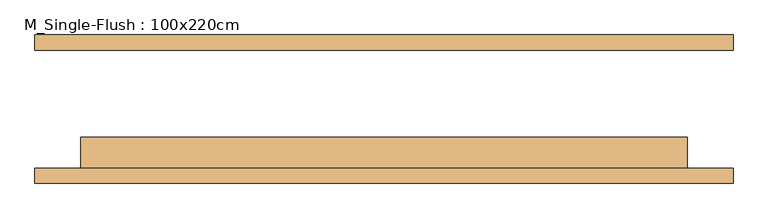
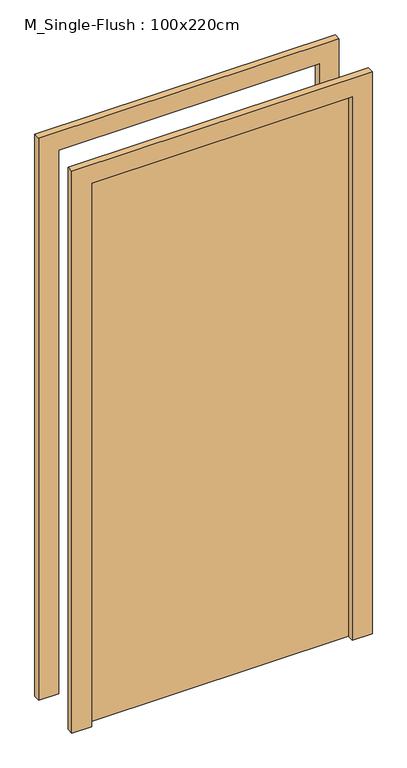
"""IFC4 building model written with IfcOpenShell, lengths in millimetres: door geometry, M_Single-Flush : 100x220cm."""

from ifc_helpers import new_model, si_unit, frame, origin, origin_with_axes, place, context, project, spatial, polyline, outline, extrude, source, transform, mapped, element, save


def m_single_flush_100x220cm_94bd71e5(model_context):
    return source(origin(), model_context, "Body", "SweptSolid", [
        extrude(outline(polyline([(2276.0, -576.0), (0.0, -576.0), (0.0, -500.0), (2200.0, -500.0), (2200.0, 500.0), (0.0, 500.0), (0.0, 576.0), (2276.0, 576.0), (2276.0, -576.0)])), frame((0.0, -122.5, 0.0), z_axis=(0.0, 1.0, 0.0), x_axis=(0.0, 0.0, 1.0)), (0.0, 0.0, 1.0), 25.0),
        extrude(outline(polyline([(2276.0, 576.0), (2276.0, -576.0), (0.0, -576.0), (0.0, -500.0), (2200.0, -500.0), (2200.0, 500.0), (0.0, 500.0), (0.0, 576.0), (2276.0, 576.0)])), frame((0.0, 97.5, 0.0), z_axis=(0.0, 1.0, 0.0), x_axis=(0.0, 0.0, 1.0)), (0.0, 0.0, 1.0), 25.0),
        extrude(outline(polyline([(500.0, -46.5), (500.0, -97.5), (-500.0, -97.5), (-500.0, -46.5), (500.0, -46.5)])), origin_with_axes(), (0.0, 0.0, 1.0), 2200.0),
    ])


if __name__ == "__main__":
    model = new_model("IFC4")
    model_context = context("Model", 3, world=origin())
    ifc_project = project(units=[si_unit("LENGTHUNIT", "METRE", prefix="MILLI")], contexts=[model_context])
    site = spatial("IfcSite", under=ifc_project)
    building = spatial("IfcBuilding", under=site)
    placement = place(None, origin())
    m_single_flush_100x220cm_shape = m_single_flush_100x220cm_94bd71e5(model_context)
    element("IfcDoor", 1, ObjectType="M_Single-Flush : 100x220cm", at=placement, inside=building, context=model_context, shape_type="MappedRepresentation", body=[
        mapped(m_single_flush_100x220cm_shape, transform((0.0, 0.0, 0.0), x_axis=(1.0, 0.0, 0.0), y_axis=(0.0, 1.0, 0.0), z_axis=(0.0, 0.0, 1.0))),
    ])
    save(model, "model.ifc")

# Revit data of these elements
# Type "M_Single-Flush : 100x220cm"
#   Type Mark = "44"
#   Construction Type Id = "MDOOR"
#   Analytic Construction = "Metal"
#   Thickness = 5.10 cm
#   Heat Transfer Coefficient (U) = 3.7021 W/(m²·K)
#   Height = 220.00 cm
#   Trim Projection Ext = 2.50 cm
#   Trim Projection Int = 2.50 cm
#   Trim Width = 7.60 cm
#   Width = 100.00 cm
#   Define Thermal Properties by = 1
#   Door Material = Door - Panel
#   Frame Material = Door - Frame
#   Visual Light Transmittance = 0
#   Solar Heat Gain Coefficient = 0
#   Function = (empty or 0)
#   Wall Closure = (empty or 0)
# Element 1 (IfcDoor, "M_Single-Flush : 100x220cm")
#   Materials on its faces: "Door - Frame", "Door - Panel"
# Materials
#   "Door - Panel": class "Wood", colour RGB 210 159 95, transparency 0, Cost = 0
#   "Door - Frame": class "Miscellaneous", colour RGB 118 70 51, transparency 0, Cost = 0
